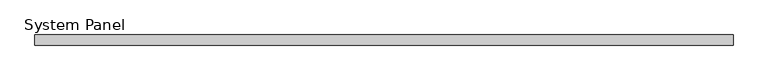
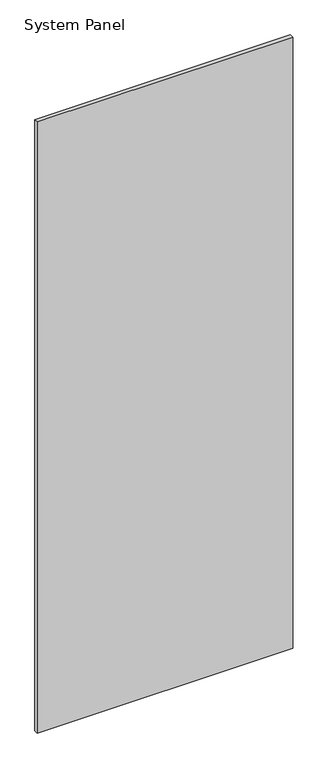
"""IFC4 building model written with IfcOpenShell, lengths in millimetres: plate geometry, System Panel : WWm-Glass-20mm-10mmOffset."""

import ifcopenshell
import ifcopenshell.guid

model = None  # the IFC model being written
_history = None  # IfcOwnerHistory: only IFC2X3 demands one
_inside = {}  # id of a spatial element -> (the spatial element, [elements in it])
_under = {}  # id of a project, library or spatial element -> (it, [spatial elements below it])
_declared = {}  # id of a project -> (the project, [libraries it declares])
_typed = {}  # id of a type object -> (the type object, [elements of that type])
_made_of = {}  # id of a material, layer set ... -> (it, [elements and type objects made of it])


def new_model(schema):
    """Start an empty IFC model of exactly this schema.

    Asked for "IFC4X3", IfcOpenShell would pick the latest addendum, in which some entities
    have other attributes; the version numbers below select the first issue.
    IFC2X3 requires an IfcOwnerHistory on every rooted entity: one is made here for all.
    """
    global model, _history
    if schema == "IFC4X3":
        model = ifcopenshell.file(schema_version=(4, 3, 0, 0))
    else:
        model = ifcopenshell.file(schema=schema)
    _inside.clear()
    _under.clear()
    _declared.clear()
    _typed.clear()
    _made_of.clear()
    _history = None
    if model.schema == "IFC2X3":
        org = make("IfcOrganization", Name="unknown")
        user = make(
            "IfcPersonAndOrganization",
            ThePerson=make("IfcPerson", FamilyName="unknown"),
            TheOrganization=org,
        )
        app = make(
            "IfcApplication",
            ApplicationDeveloper=org,
            Version="unknown",
            ApplicationFullName="unknown",
            ApplicationIdentifier="unknown",
        )
        _history = make(
            "IfcOwnerHistory",
            OwningUser=user,
            OwningApplication=app,
            ChangeAction="ADDED",
            CreationDate=0,
        )
    return model


def make(cls, **values):
    """One entity of the class cls with the attributes given. An attribute that is None is left unset."""
    return model.create_entity(
        cls, **{name: value for name, value in values.items() if value is not None}
    )


def rooted(cls, **values):
    """An entity with a GlobalId (a new one), such as an element, a storey or a relation."""
    return make(cls, GlobalId=ifcopenshell.guid.new(), OwnerHistory=_history, **values)


def si_unit(unit_type, name, prefix=None):
    """IfcSIUnit, for example si_unit("LENGTHUNIT", "METRE", prefix="MILLI")."""
    return make("IfcSIUnit", UnitType=unit_type, Prefix=prefix, Name=name)


def assignment(units):
    """IfcUnitAssignment: the units of a project."""
    return None if units is None else make("IfcUnitAssignment", Units=units)


def point(xyz):
    """IfcCartesianPoint."""
    return None if xyz is None else make("IfcCartesianPoint", Coordinates=xyz)


def direction(xyz):
    """IfcDirection."""
    return None if xyz is None else make("IfcDirection", DirectionRatios=xyz)


def frame(location, z_axis=None, x_axis=None):
    """IfcAxis2Placement3D, a coordinate frame: its origin and axes. An axis left out is left unset."""
    return make(
        "IfcAxis2Placement3D",
        Location=point(location),
        Axis=direction(z_axis),
        RefDirection=direction(x_axis),
    )


def origin():
    """The frame at (0, 0, 0) with its axes left unset."""
    return frame((0.0, 0.0, 0.0))


def origin_with_axes():
    """The frame at (0, 0, 0) with the z axis (0, 0, 1) and the x axis (1, 0, 0) written out."""
    return frame((0.0, 0.0, 0.0), z_axis=(0.0, 0.0, 1.0), x_axis=(1.0, 0.0, 0.0))


def place(relative_to, where):
    """IfcLocalPlacement: puts the frame where relative to a parent placement (None: the world)."""
    return make(
        "IfcLocalPlacement", PlacementRelTo=relative_to, RelativePlacement=where
    )


def context(
    kind, dimensions, precision=None, world=None, true_north=None, identifier=None
):
    """IfcGeometricRepresentationContext, for example the 3D "Model" context."""
    return make(
        "IfcGeometricRepresentationContext",
        ContextIdentifier=identifier,
        ContextType=kind,
        CoordinateSpaceDimension=dimensions,
        Precision=precision,
        WorldCoordinateSystem=world,
        TrueNorth=true_north,
    )


def project(units=None, contexts=None):
    """IfcProject with its units and contexts."""
    return rooted(
        "IfcProject",
        Name="project",
        RepresentationContexts=contexts,
        UnitsInContext=assignment(units),
    )


def spatial(cls, under=None, at=None, **own):
    """A site, building, storey or space (cls), placed at a placement, below another one or the project."""
    s = rooted(cls, ObjectPlacement=at, **own)
    if under is not None:
        _under.setdefault(under.id(), (under, []))[1].append(s)
    return s


def polyline(points):
    """IfcPolyline through the points."""
    return make("IfcPolyline", Points=[point(p) for p in points])


def outline(outer, holes=None, kind="AREA"):
    """IfcArbitraryClosedProfileDef: a profile drawn as a closed curve; with holes, ...WithVoids."""
    if holes is None:
        return make("IfcArbitraryClosedProfileDef", ProfileType=kind, OuterCurve=outer)
    return make(
        "IfcArbitraryProfileDefWithVoids",
        ProfileType=kind,
        OuterCurve=outer,
        InnerCurves=holes,
    )


def extrude(swept, where, along, depth):
    """IfcExtrudedAreaSolid: the profile swept, set in the frame where, extruded along a direction by depth."""
    return make(
        "IfcExtrudedAreaSolid",
        SweptArea=swept,
        Position=where,
        ExtrudedDirection=direction(along),
        Depth=depth,
    )


def shape(context_of_items, identifier, shape_type, items):
    """IfcShapeRepresentation: the items that make up one representation, for example the "Body"."""
    return make(
        "IfcShapeRepresentation",
        ContextOfItems=context_of_items,
        RepresentationIdentifier=identifier,
        RepresentationType=shape_type,
        Items=items,
    )


def source(mapping_origin, context_of_items, identifier, shape_type, items):
    """IfcRepresentationMap: a shape defined once, which mapped items show again and again."""
    return make(
        "IfcRepresentationMap",
        MappingOrigin=mapping_origin,
        MappedRepresentation=shape(context_of_items, identifier, shape_type, items),
    )


def transform(
    local_origin,
    x_axis=None,
    y_axis=None,
    z_axis=None,
    scale=None,
    scale2=None,
    scale3=None,
    uniform=True,
):
    """IfcCartesianTransformationOperator3D, or its non-uniform kind. x_axis, y_axis, z_axis: its Axis1, 2, 3."""
    if uniform:
        return make(
            "IfcCartesianTransformationOperator3D",
            Axis1=direction(x_axis),
            Axis2=direction(y_axis),
            LocalOrigin=point(local_origin),
            Scale=scale,
            Axis3=direction(z_axis),
        )
    return make(
        "IfcCartesianTransformationOperator3DnonUniform",
        Axis1=direction(x_axis),
        Axis2=direction(y_axis),
        LocalOrigin=point(local_origin),
        Scale=scale,
        Axis3=direction(z_axis),
        Scale2=scale2,
        Scale3=scale3,
    )


def mapped(mapping_source, mapping_target):
    """IfcMappedItem: shows the shape of a source again, moved by a transform."""
    return make(
        "IfcMappedItem", MappingSource=mapping_source, MappingTarget=mapping_target
    )


def made_of(thing, what):
    """Note that an element or type object is made of a material, layer set ...; save() writes the relation."""
    if what is not None:
        _made_of.setdefault(what.id(), (what, []))[1].append(thing)
    return thing


def element(
    cls,
    number,
    at=None,
    inside=None,
    cuts=None,
    type_object=None,
    material=None,
    context=None,
    identifier="Body",
    shape_type=None,
    held_by="IfcProductDefinitionShape",
    body=None,
    shapes=None,
    **own,
):
    """One element of the class cls, such as IfcWall. Its Tag is "e" and its number.

    at: its placement. inside: the storey or other place that contains it. cuts: it is an
    opening in that element (IfcRelVoidsElement). A single representation is given by context,
    identifier, shape_type and body (its items); several are given by shapes. held_by: the class
    of the entity that holds the representations. save() writes the other relations.
    """
    e = rooted(cls, Tag="e%d" % number, ObjectPlacement=at, **own)
    if body is not None:
        shapes = [shape(context, identifier, shape_type, body)]
    if shapes is not None:
        e.Representation = make(held_by, Representations=shapes)
    if inside is not None:
        _inside.setdefault(inside.id(), (inside, []))[1].append(e)
    if cuts is not None:
        rooted(
            "IfcRelVoidsElement", RelatingBuildingElement=cuts, RelatedOpeningElement=e
        )
    if type_object is not None:
        _typed.setdefault(type_object.id(), (type_object, []))[1].append(e)
    return made_of(e, material)


def aggregate(whole, parts):
    """IfcRelAggregates: a whole, such as a stair, and the parts it consists of."""
    return rooted("IfcRelAggregates", RelatingObject=whole, RelatedObjects=parts)


def save(model, path):
    """Write the relations noted so far, then the file.

    IfcRelAggregates (storeys below a building ...), IfcRelContainedInSpatialStructure (elements
    in a storey), IfcRelDefinesByType, IfcRelAssociatesMaterial and IfcRelDeclares: one each for
    every whole, place, type object, material and project.
    """
    for whole, parts in _under.values():
        aggregate(whole, parts)
    for where, things in _inside.values():
        rooted(
            "IfcRelContainedInSpatialStructure",
            RelatedElements=things,
            RelatingStructure=where,
        )
    for kind, things in _typed.values():
        rooted("IfcRelDefinesByType", RelatedObjects=things, RelatingType=kind)
    for what, things in _made_of.values():
        rooted("IfcRelAssociatesMaterial", RelatedObjects=things, RelatingMaterial=what)
    for by, libraries in _declared.values():
        rooted("IfcRelDeclares", RelatingContext=by, RelatedDefinitions=libraries)
    model.write(path)


def system_panel_029e3139(model_context):
    return source(origin(), model_context, "Body", "SweptSolid", [
        extrude(outline(polyline([(662.0016843, 0.0), (-662.0016843, 0.0), (-662.0016843, 20.0), (662.0016843, 20.0), (662.0016843, 0.0)])), origin_with_axes(), (0.0, 0.0, 1.0), 3350.0),
    ])


if __name__ == "__main__":
    model = new_model("IFC4")
    model_context = context("Model", 3, world=origin())
    ifc_project = project(units=[si_unit("LENGTHUNIT", "METRE", prefix="MILLI")], contexts=[model_context])
    site = spatial("IfcSite", under=ifc_project)
    building = spatial("IfcBuilding", under=site)
    placement = place(None, origin())
    system_panel_shape = system_panel_029e3139(model_context)
    element("IfcPlate", 1, ObjectType="System Panel : WWm-Glass-20mm-10mmOffset", at=placement, inside=building, context=model_context, shape_type="MappedRepresentation", body=[
        mapped(system_panel_shape, transform((0.0, 0.0, 0.0), x_axis=(1.0, 0.0, 0.0), y_axis=(0.0, 1.0, 0.0), z_axis=(0.0, 0.0, 1.0))),
    ])
    save(model, "model.ifc")

# Revit data of these elements
# Type "System Panel : WWm-Glass-20mm-10mmOffset"
#   Finish = ""
# Element 1 (IfcPlate, "System Panel : WWm-Glass-20mm-10mmOffset")
#   Materials on its faces: "WW-EC-GL-Storefront"
# Materials
#   "WW-EC-GL-Storefront": class "Glass", colour RGB 236 240 239, transparency 0.85, Description = "Storefront Glass", Cost = 0
